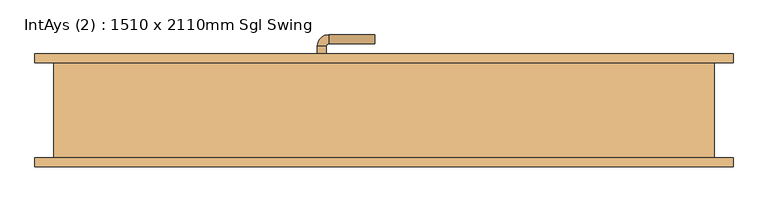
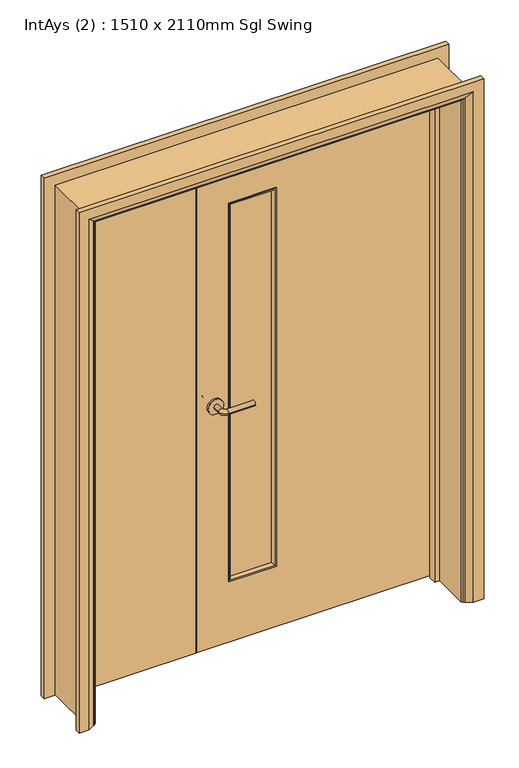
"""IFC4 building model written with IfcOpenShell, lengths in millimetres: door geometry, IntAys (2) : 1510 x 2110mm Sgl Swing."""

import ifcopenshell
import ifcopenshell.guid

model = None  # the IFC model being written
_history = None  # IfcOwnerHistory: only IFC2X3 demands one
_inside = {}  # id of a spatial element -> (the spatial element, [elements in it])
_under = {}  # id of a project, library or spatial element -> (it, [spatial elements below it])
_declared = {}  # id of a project -> (the project, [libraries it declares])
_typed = {}  # id of a type object -> (the type object, [elements of that type])
_made_of = {}  # id of a material, layer set ... -> (it, [elements and type objects made of it])


def new_model(schema):
    """Start an empty IFC model of exactly this schema.

    Asked for "IFC4X3", IfcOpenShell would pick the latest addendum, in which some entities
    have other attributes; the version numbers below select the first issue.
    IFC2X3 requires an IfcOwnerHistory on every rooted entity: one is made here for all.
    """
    global model, _history
    if schema == "IFC4X3":
        model = ifcopenshell.file(schema_version=(4, 3, 0, 0))
    else:
        model = ifcopenshell.file(schema=schema)
    _inside.clear()
    _under.clear()
    _declared.clear()
    _typed.clear()
    _made_of.clear()
    _history = None
    if model.schema == "IFC2X3":
        org = make("IfcOrganization", Name="unknown")
        user = make(
            "IfcPersonAndOrganization",
            ThePerson=make("IfcPerson", FamilyName="unknown"),
            TheOrganization=org,
        )
        app = make(
            "IfcApplication",
            ApplicationDeveloper=org,
            Version="unknown",
            ApplicationFullName="unknown",
            ApplicationIdentifier="unknown",
        )
        _history = make(
            "IfcOwnerHistory",
            OwningUser=user,
            OwningApplication=app,
            ChangeAction="ADDED",
            CreationDate=0,
        )
    return model


def make(cls, **values):
    """One entity of the class cls with the attributes given. An attribute that is None is left unset."""
    return model.create_entity(
        cls, **{name: value for name, value in values.items() if value is not None}
    )


def rooted(cls, **values):
    """An entity with a GlobalId (a new one), such as an element, a storey or a relation."""
    return make(cls, GlobalId=ifcopenshell.guid.new(), OwnerHistory=_history, **values)


def si_unit(unit_type, name, prefix=None):
    """IfcSIUnit, for example si_unit("LENGTHUNIT", "METRE", prefix="MILLI")."""
    return make("IfcSIUnit", UnitType=unit_type, Prefix=prefix, Name=name)


def assignment(units):
    """IfcUnitAssignment: the units of a project."""
    return None if units is None else make("IfcUnitAssignment", Units=units)


def point(xyz):
    """IfcCartesianPoint."""
    return None if xyz is None else make("IfcCartesianPoint", Coordinates=xyz)


def direction(xyz):
    """IfcDirection."""
    return None if xyz is None else make("IfcDirection", DirectionRatios=xyz)


def frame(location, z_axis=None, x_axis=None):
    """IfcAxis2Placement3D, a coordinate frame: its origin and axes. An axis left out is left unset."""
    return make(
        "IfcAxis2Placement3D",
        Location=point(location),
        Axis=direction(z_axis),
        RefDirection=direction(x_axis),
    )


def frame_2d(location, x_axis=None):
    """IfcAxis2Placement2D, a coordinate frame in the plane: its origin and x axis."""
    return make(
        "IfcAxis2Placement2D", Location=point(location), RefDirection=direction(x_axis)
    )


def origin():
    """The frame at (0, 0, 0) with its axes left unset."""
    return frame((0.0, 0.0, 0.0))


def place(relative_to, where):
    """IfcLocalPlacement: puts the frame where relative to a parent placement (None: the world)."""
    return make(
        "IfcLocalPlacement", PlacementRelTo=relative_to, RelativePlacement=where
    )


def context(
    kind, dimensions, precision=None, world=None, true_north=None, identifier=None
):
    """IfcGeometricRepresentationContext, for example the 3D "Model" context."""
    return make(
        "IfcGeometricRepresentationContext",
        ContextIdentifier=identifier,
        ContextType=kind,
        CoordinateSpaceDimension=dimensions,
        Precision=precision,
        WorldCoordinateSystem=world,
        TrueNorth=true_north,
    )


def project(units=None, contexts=None):
    """IfcProject with its units and contexts."""
    return rooted(
        "IfcProject",
        Name="project",
        RepresentationContexts=contexts,
        UnitsInContext=assignment(units),
    )


def spatial(cls, under=None, at=None, **own):
    """A site, building, storey or space (cls), placed at a placement, below another one or the project."""
    s = rooted(cls, ObjectPlacement=at, **own)
    if under is not None:
        _under.setdefault(under.id(), (under, []))[1].append(s)
    return s


def polyline(points):
    """IfcPolyline through the points."""
    return make("IfcPolyline", Points=[point(p) for p in points])


def circle_curve(where, radius):
    """IfcCircle in the frame where."""
    return make("IfcCircle", Position=where, Radius=radius)


def ellipse_curve(where, semi_axis1, semi_axis2):
    """IfcEllipse in the frame where."""
    return make(
        "IfcEllipse", Position=where, SemiAxis1=semi_axis1, SemiAxis2=semi_axis2
    )


def trimmed(basis, trim1, trim2, sense, master):
    """IfcTrimmedCurve: the piece of a basis curve between two trims."""
    return make(
        "IfcTrimmedCurve",
        BasisCurve=basis,
        Trim1=trim1,
        Trim2=trim2,
        SenseAgreement=sense,
        MasterRepresentation=master,
    )


def segment(curve, same_sense, transition):
    """IfcCompositeCurveSegment."""
    return make(
        "IfcCompositeCurveSegment",
        Transition=transition,
        SameSense=same_sense,
        ParentCurve=curve,
    )


def composite_curve(segments, self_intersect=None):
    """IfcCompositeCurve: segments joined end to end."""
    return make("IfcCompositeCurve", Segments=segments, SelfIntersect=self_intersect)


def outline(outer, holes=None, kind="AREA"):
    """IfcArbitraryClosedProfileDef: a profile drawn as a closed curve; with holes, ...WithVoids."""
    if holes is None:
        return make("IfcArbitraryClosedProfileDef", ProfileType=kind, OuterCurve=outer)
    return make(
        "IfcArbitraryProfileDefWithVoids",
        ProfileType=kind,
        OuterCurve=outer,
        InnerCurves=holes,
    )


def extrude(swept, where, along, depth):
    """IfcExtrudedAreaSolid: the profile swept, set in the frame where, extruded along a direction by depth."""
    return make(
        "IfcExtrudedAreaSolid",
        SweptArea=swept,
        Position=where,
        ExtrudedDirection=direction(along),
        Depth=depth,
    )


def faces_of(points, faces, orient=None, outer=None):
    """IfcFace entities. A face is a list of loops; a loop is a list of indices into points, from 0.

    orient and outer hold one flag for each loop. By default every Orientation is true, the
    first loop of a face is its IfcFaceOuterBound and the others are IfcFaceBound.
    """
    made = []
    for i, loops in enumerate(faces):
        bounds = []
        for j, loop in enumerate(loops):
            is_outer = j == 0 if outer is None else outer[i][j]
            bounds.append(
                make(
                    "IfcFaceOuterBound" if is_outer else "IfcFaceBound",
                    Bound=make("IfcPolyLoop", Polygon=[points[k] for k in loop]),
                    Orientation=True if orient is None else orient[i][j],
                )
            )
        made.append(make("IfcFace", Bounds=bounds))
    return made


def faceted_brep(points, faces, orient=None, outer=None, voids=None):
    """IfcFacetedBrep: a solid bounded by flat faces; with voids (closed shells), ...WithVoids."""
    shared = [point(p) for p in points]
    hull = make("IfcClosedShell", CfsFaces=faces_of(shared, faces, orient, outer))
    if voids is None:
        return make("IfcFacetedBrep", Outer=hull)
    return make(
        "IfcFacetedBrepWithVoids",
        Outer=hull,
        Voids=[
            make(cls, CfsFaces=faces_of(shared, fs, o, b)) for cls, fs, o, b in voids
        ],
    )


def shape(context_of_items, identifier, shape_type, items):
    """IfcShapeRepresentation: the items that make up one representation, for example the "Body"."""
    return make(
        "IfcShapeRepresentation",
        ContextOfItems=context_of_items,
        RepresentationIdentifier=identifier,
        RepresentationType=shape_type,
        Items=items,
    )


def source(mapping_origin, context_of_items, identifier, shape_type, items):
    """IfcRepresentationMap: a shape defined once, which mapped items show again and again."""
    return make(
        "IfcRepresentationMap",
        MappingOrigin=mapping_origin,
        MappedRepresentation=shape(context_of_items, identifier, shape_type, items),
    )


def transform(
    local_origin,
    x_axis=None,
    y_axis=None,
    z_axis=None,
    scale=None,
    scale2=None,
    scale3=None,
    uniform=True,
):
    """IfcCartesianTransformationOperator3D, or its non-uniform kind. x_axis, y_axis, z_axis: its Axis1, 2, 3."""
    if uniform:
        return make(
            "IfcCartesianTransformationOperator3D",
            Axis1=direction(x_axis),
            Axis2=direction(y_axis),
            LocalOrigin=point(local_origin),
            Scale=scale,
            Axis3=direction(z_axis),
        )
    return make(
        "IfcCartesianTransformationOperator3DnonUniform",
        Axis1=direction(x_axis),
        Axis2=direction(y_axis),
        LocalOrigin=point(local_origin),
        Scale=scale,
        Axis3=direction(z_axis),
        Scale2=scale2,
        Scale3=scale3,
    )


def mapped(mapping_source, mapping_target):
    """IfcMappedItem: shows the shape of a source again, moved by a transform."""
    return make(
        "IfcMappedItem", MappingSource=mapping_source, MappingTarget=mapping_target
    )


def made_of(thing, what):
    """Note that an element or type object is made of a material, layer set ...; save() writes the relation."""
    if what is not None:
        _made_of.setdefault(what.id(), (what, []))[1].append(thing)
    return thing


def element(
    cls,
    number,
    at=None,
    inside=None,
    cuts=None,
    type_object=None,
    material=None,
    context=None,
    identifier="Body",
    shape_type=None,
    held_by="IfcProductDefinitionShape",
    body=None,
    shapes=None,
    **own,
):
    """One element of the class cls, such as IfcWall. Its Tag is "e" and its number.

    at: its placement. inside: the storey or other place that contains it. cuts: it is an
    opening in that element (IfcRelVoidsElement). A single representation is given by context,
    identifier, shape_type and body (its items); several are given by shapes. held_by: the class
    of the entity that holds the representations. save() writes the other relations.
    """
    e = rooted(cls, Tag="e%d" % number, ObjectPlacement=at, **own)
    if body is not None:
        shapes = [shape(context, identifier, shape_type, body)]
    if shapes is not None:
        e.Representation = make(held_by, Representations=shapes)
    if inside is not None:
        _inside.setdefault(inside.id(), (inside, []))[1].append(e)
    if cuts is not None:
        rooted(
            "IfcRelVoidsElement", RelatingBuildingElement=cuts, RelatedOpeningElement=e
        )
    if type_object is not None:
        _typed.setdefault(type_object.id(), (type_object, []))[1].append(e)
    return made_of(e, material)


def aggregate(whole, parts):
    """IfcRelAggregates: a whole, such as a stair, and the parts it consists of."""
    return rooted("IfcRelAggregates", RelatingObject=whole, RelatedObjects=parts)


def save(model, path):
    """Write the relations noted so far, then the file.

    IfcRelAggregates (storeys below a building ...), IfcRelContainedInSpatialStructure (elements
    in a storey), IfcRelDefinesByType, IfcRelAssociatesMaterial and IfcRelDeclares: one each for
    every whole, place, type object, material and project.
    """
    for whole, parts in _under.values():
        aggregate(whole, parts)
    for where, things in _inside.values():
        rooted(
            "IfcRelContainedInSpatialStructure",
            RelatedElements=things,
            RelatingStructure=where,
        )
    for kind, things in _typed.values():
        rooted("IfcRelDefinesByType", RelatedObjects=things, RelatingType=kind)
    for what, things in _made_of.values():
        rooted("IfcRelAssociatesMaterial", RelatedObjects=things, RelatingMaterial=what)
    for by, libraries in _declared.values():
        rooted("IfcRelDeclares", RelatingContext=by, RelatedDefinitions=libraries)
    model.write(path)


def plane_surface(at):
    """IfcPlane: the flat surface through the origin of the frame at, square to its z axis."""
    return make("IfcPlane", Position=at)


def cylinder_surface(at, radius):
    """IfcCylindricalSurface: all points at the distance radius from the z axis of the frame at."""
    return make("IfcCylindricalSurface", Position=at, Radius=radius)


def revolved_surface(curve, axis_point, axis_direction):
    """IfcSurfaceOfRevolution: the curve turned about the line through axis_point along axis_direction."""
    return make(
        "IfcSurfaceOfRevolution",
        SweptCurve=make("IfcArbitraryOpenProfileDef", ProfileType="CURVE", Curve=curve),
        AxisPosition=make("IfcAxis1Placement", Location=point(axis_point), Axis=direction(axis_direction)),
    )


def advanced_brep(points, edges, surfaces, faces):
    """IfcAdvancedBrep: a solid bounded by faces that lie on surfaces and meet in shared edges.

    An edge is (start, end): straight between two places in points (the first is 0);
    or (start, end, curve); or (start, end, curve, False) where it runs against its curve.
    A face is (place in surfaces, loops), or (place, loops, False) where it looks against
    its surface's normal. A loop lists edges by number (the first is 1), with a minus sign
    where the edge is run from its end to its start. The first loop is the outer one.
    """
    corners = [point(p) for p in points]
    vertices = [make("IfcVertexPoint", VertexGeometry=c) for c in corners]
    made = []
    for start, end, *more in edges:
        made.append(
            make(
                "IfcEdgeCurve",
                EdgeStart=vertices[start],
                EdgeEnd=vertices[end],
                EdgeGeometry=more[0] if more else make("IfcPolyline", Points=[corners[start], corners[end]]),
                SameSense=more[1] if len(more) > 1 else True,
            )
        )
    hull = []
    for where, loops, *sense in faces:
        bounds = []
        for j, loop in enumerate(loops):
            ring = [make("IfcOrientedEdge", EdgeElement=made[abs(k) - 1], Orientation=k > 0) for k in loop]
            bounds.append(
                make(
                    "IfcFaceOuterBound" if j == 0 else "IfcFaceBound",
                    Bound=make("IfcEdgeLoop", EdgeList=ring),
                    Orientation=True,
                )
            )
        hull.append(make("IfcAdvancedFace", Bounds=bounds, FaceSurface=surfaces[where], SameSense=sense[0] if sense else True))
    return make("IfcAdvancedBrep", Outer=make("IfcClosedShell", CfsFaces=hull))


def intays_2_1510_x_2110mm_sgl_swing_d010f506(model_context):
    return source(origin(), model_context, "Body", "SolidModel", [
        advanced_brep(
        [(88.5, 67.5, 1000.0), (108.5, 67.5, 1000.0), (108.5, 37.5, 1000.0), (88.5, 37.5, 1000.0), (113.5, 32.5, 1000.0), (113.5, 12.5, 1000.0), (218.5, 12.5, 1000.0), (218.5, 32.5, 1000.0)],
        [
            (0, 1, circle_curve(frame((98.5, 67.5, 1000.0), z_axis=(0.0, 1.0, 0.0), x_axis=(1.0, 0.0, 0.0)), 10.0)),
            (1, 0, circle_curve(frame((98.5, 67.5, 1000.0), z_axis=(0.0, 1.0, 0.0), x_axis=(1.0, 0.0, 0.0)), 10.0)),
            (1, 2),
            (2, 3, circle_curve(frame((98.5, 37.5, 1000.0), z_axis=(0.0, 1.0, 0.0), x_axis=(1.0, 0.0, 0.0)), 10.0)),
            (3, 0),
            (3, 2, circle_curve(frame((98.5, 37.5, 1000.0), z_axis=(0.0, 1.0, 0.0), x_axis=(1.0, 0.0, 0.0)), 10.0)),
            (4, 5, circle_curve(frame((113.5, 22.5, 1000.0), z_axis=(-1.0, 0.0, 0.0), x_axis=(0.0, 1.0, 0.0)), 10.0)),
            (5, 3, circle_curve(frame((113.5, 37.5, 1000.0), z_axis=(0.0, 0.0, -1.0), x_axis=(-1.0, 0.0, 0.0)), 25.0)),
            (2, 4, circle_curve(frame((113.5, 37.5, 1000.0), z_axis=(0.0, 0.0, 1.0), x_axis=(-1.0, 0.0, 0.0)), 5.0)),
            (5, 4, circle_curve(frame((113.5, 22.5, 1000.0), z_axis=(-1.0, 0.0, 0.0), x_axis=(0.0, 1.0, 0.0)), 10.0)),
            (6, 7, circle_curve(frame((218.5, 22.5, 1000.0), z_axis=(1.0, 0.0, 0.0), x_axis=(0.0, 1.0, 0.0)), 10.0)),
            (7, 6, circle_curve(frame((218.5, 22.5, 1000.0), z_axis=(1.0, 0.0, 0.0), x_axis=(0.0, 1.0, 0.0)), 10.0)),
            (4, 7),
            (6, 5),
        ],
        [
            plane_surface(frame((98.5, 67.5, 1000.0), z_axis=(0.0, 1.0, 0.0), x_axis=(0.0, 0.0, 1.0))),
            cylinder_surface(frame((98.5, 67.5, 1000.0), z_axis=(0.0, 1.0, 0.0), x_axis=(1.0, 0.0, 0.0)), 10.0),
            revolved_surface(trimmed(ellipse_curve(frame((98.5, 37.5, 1000.0), z_axis=(0.0, -1.0, 0.0), x_axis=(1.0, 0.0, 0.0)), 10.0, 10.0), [point((88.5, 37.5, 1000.0))], [point((108.5, 37.5, 1000.0))], True, "CARTESIAN"), (113.5, 37.5, 1000.0), (0.0, 0.0, -1.0)),
            revolved_surface(trimmed(ellipse_curve(frame((98.5, 37.5, 1000.0), z_axis=(0.0, -1.0, 0.0), x_axis=(1.0, 0.0, 0.0)), 10.0, 10.0), [point((108.5, 37.5, 1000.0))], [point((88.5, 37.5, 1000.0))], True, "CARTESIAN"), (113.5, 37.5, 1000.0), (0.0, 0.0, -1.0)),
            plane_surface(frame((218.5, 22.5, 1000.0), z_axis=(1.0, 0.0, 0.0), x_axis=(0.0, 0.0, 1.0))),
            cylinder_surface(frame((113.5, 22.5, 1000.0), z_axis=(-1.0, 0.0, 0.0), x_axis=(0.0, 1.0, 0.0)), 10.0),
        ],
        [
            (0, [[1, 2]]),
            (1, [[3, 4, 5, -2]]),
            (1, [[-5, 6, -3, -1]]),
            (2, [[7, 8, -4, 9]]),
            (3, [[10, -9, -6, -8]]),
            (4, [[11, 12]]),
            (5, [[13, -11, 14, -7]]),
            (5, [[-14, -12, -13, -10]]),
        ],
    ),
        extrude(outline(composite_curve([segment(trimmed(circle_curve(frame_2d((1000.0, 96.0)), 30.0), [point((1000.0, 66.0))], [point((1000.0, 126.0))], False, "CARTESIAN"), True, "CONTINUOUS"), segment(trimmed(circle_curve(frame_2d((1000.0, 96.0)), 30.0), [point((1000.0, 126.0))], [point((1000.0, 66.0))], False, "CARTESIAN"), True, "CONTINUOUS")], self_intersect=False)), frame((0.0, 67.5, 0.0), z_axis=(0.0, 1.0, 0.0), x_axis=(0.0, 0.0, 1.0)), (0.0, 0.0, 1.0), 8.0),
        advanced_brep(
        [(88.5, 115.5, 1000.0), (108.5, 115.5, 1000.0), (88.5, 145.5, 1000.0), (108.5, 145.5, 1000.0), (113.5, 150.5, 1000.0), (113.5, 170.5, 1000.0), (218.5, 170.5, 1000.0), (218.5, 150.5, 1000.0)],
        [
            (0, 1, circle_curve(frame((98.5, 115.5, 1000.0), z_axis=(0.0, -1.0, 0.0), x_axis=(1.0, 0.0, 0.0)), 10.0)),
            (1, 0, circle_curve(frame((98.5, 115.5, 1000.0), z_axis=(0.0, -1.0, 0.0), x_axis=(1.0, 0.0, 0.0)), 10.0)),
            (0, 2),
            (2, 3, circle_curve(frame((98.5, 145.5, 1000.0), z_axis=(0.0, -1.0, 0.0), x_axis=(1.0, 0.0, 0.0)), 10.0)),
            (3, 1),
            (3, 2, circle_curve(frame((98.5, 145.5, 1000.0), z_axis=(0.0, -1.0, 0.0), x_axis=(1.0, 0.0, 0.0)), 10.0)),
            (4, 3, circle_curve(frame((113.5, 145.5, 1000.0), z_axis=(0.0, 0.0, 1.0), x_axis=(-1.0, 0.0, 0.0)), 5.0)),
            (2, 5, circle_curve(frame((113.5, 145.5, 1000.0), z_axis=(0.0, 0.0, -1.0), x_axis=(-1.0, 0.0, 0.0)), 25.0)),
            (5, 4, circle_curve(frame((113.5, 160.5, 1000.0), z_axis=(-1.0, 0.0, 0.0), x_axis=(0.0, -1.0, 0.0)), 10.0)),
            (4, 5, circle_curve(frame((113.5, 160.5, 1000.0), z_axis=(-1.0, 0.0, 0.0), x_axis=(0.0, -1.0, 0.0)), 10.0)),
            (6, 7, circle_curve(frame((218.5, 160.5, 1000.0), z_axis=(1.0, 0.0, 0.0), x_axis=(0.0, -1.0, 0.0)), 10.0)),
            (7, 6, circle_curve(frame((218.5, 160.5, 1000.0), z_axis=(1.0, 0.0, 0.0), x_axis=(0.0, -1.0, 0.0)), 10.0)),
            (5, 6),
            (7, 4),
        ],
        [
            plane_surface(frame((98.5, 115.5, 1000.0), z_axis=(0.0, -1.0, 0.0), x_axis=(0.0, 0.0, 1.0))),
            cylinder_surface(frame((98.5, 115.5, 1000.0), z_axis=(0.0, -1.0, 0.0), x_axis=(1.0, 0.0, 0.0)), 10.0),
            revolved_surface(trimmed(ellipse_curve(frame((98.5, 145.5, 1000.0), z_axis=(0.0, -1.0, 0.0), x_axis=(1.0, 0.0, 0.0)), 10.0, 10.0), [point((88.5, 145.5, 1000.0))], [point((108.5, 145.5, 1000.0))], True, "CARTESIAN"), (113.5, 145.5, 1000.0), (0.0, 0.0, -1.0)),
            revolved_surface(trimmed(ellipse_curve(frame((98.5, 145.5, 1000.0), z_axis=(0.0, -1.0, 0.0), x_axis=(1.0, 0.0, 0.0)), 10.0, 10.0), [point((108.5, 145.5, 1000.0))], [point((88.5, 145.5, 1000.0))], True, "CARTESIAN"), (113.5, 145.5, 1000.0), (0.0, 0.0, -1.0)),
            plane_surface(frame((218.5, 160.5, 1000.0), z_axis=(1.0, 0.0, 0.0), x_axis=(0.0, 0.0, 1.0))),
            cylinder_surface(frame((113.5, 160.5, 1000.0), z_axis=(-1.0, 0.0, 0.0), x_axis=(0.0, -1.0, 0.0)), 10.0),
        ],
        [
            (0, [[1, 2]]),
            (1, [[-1, 3, 4, 5]]),
            (1, [[-2, -5, 6, -3]]),
            (2, [[7, -4, 8, 9]]),
            (3, [[-8, -6, -7, 10]]),
            (4, [[11, 12]]),
            (5, [[-9, 13, -12, 14]]),
            (5, [[-10, -14, -11, -13]]),
        ],
    ),
        extrude(outline(composite_curve([segment(trimmed(circle_curve(frame_2d((1000.0, 96.0)), 30.0), [point((1000.0, 66.0))], [point((1000.0, 126.0))], False, "CARTESIAN"), True, "CONTINUOUS"), segment(trimmed(circle_curve(frame_2d((1000.0, 96.0)), 30.0), [point((1000.0, 126.0))], [point((1000.0, 66.0))], False, "CARTESIAN"), True, "CONTINUOUS")], self_intersect=False)), frame((0.0, 107.5, 0.0), z_axis=(0.0, 1.0, 0.0), x_axis=(0.0, 0.0, 1.0)), (0.0, 0.0, 1.0), 8.0),
        extrude(outline(polyline([(2102.0, -508.0), (0.0, -508.0), (0.0, -476.0), (2070.0, -476.0), (2070.0, 954.0), (0.0, 954.0), (0.0, 986.0), (2102.0, 986.0), (2102.0, -508.0)])), frame((0.0, -107.5, 0.0), z_axis=(0.0, 1.0, 0.0), x_axis=(0.0, 0.0, 1.0)), (0.0, 0.0, 1.0), 215.0),
        advanced_brep(
        [(-551.0, -127.5, 0.0), (-551.0, -107.5, 0.0), (-481.0, -107.5, 0.0), (-485.0, -113.5, 0.0), (-511.0, -127.5, 0.0), (-551.0, -127.5, 2145.0), (-551.0, -107.5, 2145.0), (1029.0, -107.5, 2145.0), (1029.0, -107.5, 0.0), (959.0, -107.5, 0.0), (959.0, -107.5, 2075.0), (-481.0, -107.5, 2075.0), (-485.0, -113.5, 2079.0), (-511.0, -127.5, 2105.0), (989.0, -127.5, 2105.0), (989.0, -127.5, 0.0), (1029.0, -127.5, 0.0), (1029.0, -127.5, 2145.0), (963.0, -113.5, 0.0), (963.0, -113.5, 2079.0)],
        [
            (0, 1),
            (1, 2),
            (2, 3, circle_curve(frame((-489.0, -106.5, 0.0), z_axis=(0.0, 0.0, -1.0), x_axis=(-1.0, 0.0, 0.0)), 8.0622577)),
            (3, 4),
            (4, 0),
            (0, 5),
            (5, 6),
            (6, 1),
            (6, 7),
            (7, 8),
            (8, 9),
            (9, 10),
            (10, 11),
            (11, 2),
            (11, 12, ellipse_curve(frame((-489.0, -106.5, 2083.0), z_axis=(-0.7071067811865475, 0.0, -0.7071067811865475), x_axis=(0.7071067811865474, 0.0, -0.7071067811865476)), 11.4017543, 8.0622577)),
            (12, 3),
            (12, 13),
            (13, 4),
            (13, 14),
            (14, 15),
            (15, 16),
            (16, 17),
            (17, 5),
            (7, 17),
            (16, 8),
            (15, 18),
            (18, 9, circle_curve(frame((967.0, -106.5, 0.0), z_axis=(0.0, 0.0, -1.0), x_axis=(1.0, 0.0, 0.0)), 8.0622577)),
            (19, 10, ellipse_curve(frame((967.0, -106.5, 2083.0), z_axis=(0.7071067811865475, 0.0, -0.7071067811865475), x_axis=(0.7071067811865474, 0.0, 0.7071067811865476)), 11.4017543, 8.0622577)),
            (18, 19),
            (14, 19),
            (19, 12),
        ],
        [
            plane_surface(frame((-481.0, -107.5, 0.0), z_axis=(0.0, 0.0, -1.0), x_axis=(0.0, -1.0, 0.0))),
            plane_surface(frame((-551.0, -127.5, 0.0), z_axis=(-1.0, 0.0, 0.0), x_axis=(0.0, 0.0, 1.0))),
            plane_surface(frame((-551.0, -107.5, 0.0), z_axis=(0.0, 1.0, 0.0), x_axis=(0.0, 0.0, 1.0))),
            cylinder_surface(frame((-489.0, -106.5, 0.0), z_axis=(0.0, 0.0, -1.0), x_axis=(-1.0, 0.0, 0.0)), 8.0622577),
            plane_surface(frame((-485.0, -113.5, 0.0), z_axis=(0.4740998230350183, -0.8804710999221749, 0.0), x_axis=(0.0, 0.0, 1.0))),
            plane_surface(frame((-511.0, -127.5, 0.0), z_axis=(0.0, -1.0, 0.0), x_axis=(0.0, 0.0, 1.0))),
            plane_surface(frame((1029.0, -127.5, 2145.0), z_axis=(1.0, 0.0, 0.0), x_axis=(0.0, 0.0, -1.0))),
            plane_surface(frame((959.0, -107.5, 0.0), z_axis=(0.0, 0.0, -1.0), x_axis=(0.0, -1.0, 0.0))),
            cylinder_surface(frame((967.0, -106.5, 2075.0), z_axis=(0.0, 0.0, 1.0), x_axis=(1.0, 0.0, 0.0)), 8.0622577),
            plane_surface(frame((963.0, -113.5, 2079.0), z_axis=(-0.4740998230350183, -0.8804710999221749, 0.0), x_axis=(0.0, 0.0, -1.0))),
            plane_surface(frame((-551.0, -127.5, 2145.0), z_axis=(0.0, 0.0, 1.0), x_axis=(1.0, 0.0, 0.0))),
            cylinder_surface(frame((-481.0, -106.5, 2083.0), z_axis=(-1.0, 0.0, 0.0), x_axis=(0.0, 0.0, 1.0)), 8.0622577),
            plane_surface(frame((-485.0, -113.5, 2079.0), z_axis=(0.0, -0.8804710999221749, -0.4740998230350183), x_axis=(1.0, 0.0, 0.0))),
        ],
        [
            (0, [[1, 2, 3, 4, 5]]),
            (1, [[-1, 6, 7, 8]]),
            (2, [[-2, -8, 9, 10, 11, 12, 13, 14]]),
            (3, [[-3, -14, 15, 16]]),
            (4, [[-4, -16, 17, 18]]),
            (5, [[-5, -18, 19, 20, 21, 22, 23, -6]]),
            (6, [[24, -22, 25, -10]]),
            (7, [[-21, 26, 27, -11, -25]]),
            (8, [[28, -12, -27, 29]]),
            (9, [[30, -29, -26, -20]]),
            (10, [[-7, -23, -24, -9]]),
            (11, [[-15, -13, -28, 31]]),
            (12, [[-17, -31, -30, -19]]),
        ],
    ),
        advanced_brep(
        [(1029.0, 127.5, 0.0), (1029.0, 107.5, 0.0), (959.0, 107.5, 0.0), (963.0, 113.5, 0.0), (989.0, 127.5, 0.0), (1029.0, 127.5, 2145.0), (1029.0, 107.5, 2145.0), (-551.0, 107.5, 2145.0), (-551.0, 107.5, 0.0), (-481.0, 107.5, 0.0), (-481.0, 107.5, 2075.0), (959.0, 107.5, 2075.0), (963.0, 113.5, 2079.0), (989.0, 127.5, 2105.0), (-511.0, 127.5, 2105.0), (-511.0, 127.5, 0.0), (-551.0, 127.5, 0.0), (-551.0, 127.5, 2145.0), (-485.0, 113.5, 0.0), (-485.0, 113.5, 2079.0)],
        [
            (0, 1),
            (1, 2),
            (2, 3, circle_curve(frame((967.0, 106.5, 0.0), z_axis=(0.0, 0.0, -1.0), x_axis=(1.0, 0.0, 0.0)), 8.0622577)),
            (3, 4),
            (4, 0),
            (0, 5),
            (5, 6),
            (6, 1),
            (6, 7),
            (7, 8),
            (8, 9),
            (9, 10),
            (10, 11),
            (11, 2),
            (11, 12, ellipse_curve(frame((967.0, 106.5, 2083.0), z_axis=(0.7071067811865475, 0.0, -0.7071067811865475), x_axis=(-0.7071067811865474, 0.0, -0.7071067811865476)), 11.4017543, 8.0622577)),
            (12, 3),
            (12, 13),
            (13, 4),
            (13, 14),
            (14, 15),
            (15, 16),
            (16, 17),
            (17, 5),
            (7, 17),
            (16, 8),
            (15, 18),
            (18, 9, circle_curve(frame((-489.0, 106.5, 0.0), z_axis=(0.0, 0.0, -1.0), x_axis=(-1.0, 0.0, 0.0)), 8.0622577)),
            (19, 10, ellipse_curve(frame((-489.0, 106.5, 2083.0), z_axis=(-0.7071067811865475, 0.0, -0.7071067811865475), x_axis=(-0.7071067811865474, 0.0, 0.7071067811865476)), 11.4017543, 8.0622577)),
            (18, 19),
            (14, 19),
            (19, 12),
        ],
        [
            plane_surface(frame((959.0, 107.5, 0.0), z_axis=(0.0, 0.0, -1.0), x_axis=(0.0, -1.0, 0.0))),
            plane_surface(frame((1029.0, 127.5, 0.0), z_axis=(1.0, 0.0, 0.0), x_axis=(0.0, 0.0, 1.0))),
            plane_surface(frame((1029.0, 107.5, 0.0), z_axis=(0.0, -1.0, 0.0), x_axis=(0.0, 0.0, 1.0))),
            cylinder_surface(frame((967.0, 106.5, 0.0), z_axis=(0.0, 0.0, -1.0), x_axis=(1.0, 0.0, 0.0)), 8.0622577),
            plane_surface(frame((963.0, 113.5, 0.0), z_axis=(-0.4740998230350126, 0.8804710999221779, 0.0), x_axis=(0.0, 0.0, 1.0))),
            plane_surface(frame((989.0, 127.5, 0.0), z_axis=(0.0, 1.0, 0.0), x_axis=(0.0, 0.0, 1.0))),
            plane_surface(frame((-551.0, 127.5, 2145.0), z_axis=(-1.0, 0.0, 0.0), x_axis=(0.0, 0.0, -1.0))),
            plane_surface(frame((-481.0, 107.5, 0.0), z_axis=(0.0, 0.0, -1.0), x_axis=(0.0, -1.0, 0.0))),
            cylinder_surface(frame((-489.0, 106.5, 2075.0), z_axis=(0.0, 0.0, 1.0), x_axis=(-1.0, 0.0, 0.0)), 8.0622577),
            plane_surface(frame((-485.0, 113.5, 2079.0), z_axis=(0.4740998230350183, 0.8804710999221749, 0.0), x_axis=(0.0, 0.0, -1.0))),
            plane_surface(frame((1029.0, 127.5, 2145.0), z_axis=(0.0, 0.0, 1.0), x_axis=(-1.0, 0.0, 0.0))),
            cylinder_surface(frame((959.0, 106.5, 2083.0), z_axis=(1.0, 0.0, 0.0), x_axis=(0.0, 0.0, 1.0)), 8.0622577),
            plane_surface(frame((963.0, 113.5, 2079.0), z_axis=(0.0, 0.8804710999221763, -0.4740998230350154), x_axis=(-1.0, 0.0, 0.0))),
        ],
        [
            (0, [[1, 2, 3, 4, 5]]),
            (1, [[-1, 6, 7, 8]]),
            (2, [[-2, -8, 9, 10, 11, 12, 13, 14]]),
            (3, [[-3, -14, 15, 16]]),
            (4, [[-4, -16, 17, 18]]),
            (5, [[-5, -18, 19, 20, 21, 22, 23, -6]]),
            (6, [[24, -22, 25, -10]]),
            (7, [[-21, 26, 27, -11, -25]]),
            (8, [[28, -12, -27, 29]]),
            (9, [[30, -29, -26, -20]]),
            (10, [[-7, -23, -24, -9]]),
            (11, [[-15, -13, -28, 31]]),
            (12, [[-17, -31, -30, -19]]),
        ],
    ),
        faceted_brep([(-457.0, 72.5, 0.0), (-457.0, 40.5, 0.0), (-476.0, 40.5, 0.0), (-476.0, 72.5, 0.0), (-457.0, 72.5, 2051.0), (-457.0, 40.5, 2051.0), (-476.0, 40.5, 2070.0), (-476.0, 72.5, 2070.0), (935.0, 72.5, 0.0), (954.0, 72.5, 0.0), (954.0, 40.5, 0.0), (935.0, 40.5, 0.0), (935.0, 72.5, 2051.0), (954.0, 72.5, 2070.0), (954.0, 40.5, 2070.0), (935.0, 40.5, 2051.0)], [[[0, 1, 2, 3]], [[1, 0, 4, 5]], [[2, 1, 5, 6]], [[3, 2, 6, 7]], [[0, 3, 7, 4]], [[8, 9, 10, 11]], [[12, 13, 9, 8]], [[13, 14, 10, 9]], [[14, 15, 11, 10]], [[15, 12, 8, 11]], [[5, 4, 12, 15]], [[6, 5, 15, 14]], [[7, 6, 14, 13]], [[4, 7, 13, 12]]]),
        extrude(outline(polyline([(335.0, 85.5), (150.0, 85.5), (150.0, 97.5), (335.0, 97.5), (335.0, 85.5)])), frame((0.0, 0.0, 257.0), z_axis=(0.0, 0.0, 1.0), x_axis=(1.0, 0.0, 0.0)), (0.0, 0.0, 1.0), 1560.0),
        extrude(outline(polyline([(22.0, 75.5), (-473.0, 75.5), (-473.0, 107.5), (22.0, 107.5), (22.0, 75.5)])), frame((0.0, 0.0, 5.753223), z_axis=(0.0, 0.0, 1.0), x_axis=(1.0, 0.0, 0.0)), (0.0, 0.0, 1.0), 2061.246777),
        extrude(outline(polyline([(5.753223, 951.0), (2067.0, 951.0), (2067.0, 25.0), (5.753223, 25.0), (5.753223, 951.0)]), holes=[polyline([(1817.0, 150.0), (1817.0, 335.0), (257.0, 335.0), (257.0, 150.0), (1817.0, 150.0)])]), frame((0.0, 75.5, 0.0), z_axis=(0.0, 1.0, 0.0), x_axis=(0.0, 0.0, 1.0)), (0.0, 0.0, 1.0), 32.0),
        faceted_brep([(335.0, 72.5, 257.0), (335.0, 85.5, 257.0), (335.0, 85.5, 1817.0), (335.0, 72.5, 1817.0), (323.0, 85.5, 269.0), (329.0, 72.5, 263.0), (329.0, 72.5, 1811.0), (323.0, 85.5, 1805.0), (150.0, 85.5, 1817.0), (150.0, 72.5, 1817.0), (156.0, 72.5, 1811.0), (162.0, 85.5, 1805.0), (150.0, 85.5, 257.0), (150.0, 72.5, 257.0), (156.0, 72.5, 263.0), (162.0, 85.5, 269.0)], [[[0, 1, 2, 3]], [[4, 5, 6, 7]], [[3, 2, 8, 9]], [[7, 6, 10, 11]], [[9, 8, 12, 13]], [[11, 10, 14, 15]], [[1, 12, 8, 2], [7, 11, 15, 4]], [[13, 12, 1, 0]], [[3, 9, 13, 0], [5, 14, 10, 6]], [[15, 14, 5, 4]]]),
        faceted_brep([(150.0, 110.5, 257.0), (150.0, 97.5, 257.0), (150.0, 97.5, 1817.0), (150.0, 110.5, 1817.0), (162.0, 97.5, 269.0), (156.0, 110.5, 263.0), (156.0, 110.5, 1811.0), (162.0, 97.5, 1805.0), (335.0, 97.5, 1817.0), (335.0, 110.5, 1817.0), (329.0, 110.5, 1811.0), (323.0, 97.5, 1805.0), (335.0, 97.5, 257.0), (335.0, 110.5, 257.0), (329.0, 110.5, 263.0), (323.0, 97.5, 269.0)], [[[0, 1, 2, 3]], [[4, 5, 6, 7]], [[3, 2, 8, 9]], [[7, 6, 10, 11]], [[9, 8, 12, 13]], [[11, 10, 14, 15]], [[1, 12, 8, 2], [7, 11, 15, 4]], [[13, 12, 1, 0]], [[3, 9, 13, 0], [5, 14, 10, 6]], [[15, 14, 5, 4]]]),
    ])


if __name__ == "__main__":
    model = new_model("IFC4")
    model_context = context("Model", 3, world=origin())
    ifc_project = project(units=[si_unit("LENGTHUNIT", "METRE", prefix="MILLI")], contexts=[model_context])
    site = spatial("IfcSite", under=ifc_project)
    building = spatial("IfcBuilding", under=site)
    placement = place(None, origin())
    intays_2_1510_x_2110mm_sgl_swing_shape = intays_2_1510_x_2110mm_sgl_swing_d010f506(model_context)
    element("IfcDoor", 1, ObjectType="IntAys (2) : 1510 x 2110mm Sgl Swing", at=placement, inside=building, context=model_context, shape_type="MappedRepresentation", body=[
        mapped(intays_2_1510_x_2110mm_sgl_swing_shape, transform((0.0, 0.0, 0.0), x_axis=(1.0, 0.0, 0.0), y_axis=(0.0, 1.0, 0.0), z_axis=(0.0, 0.0, 1.0))),
    ])
    save(model, "model.ifc")

# Revit data of these elements
# Type "IntAys (2) : 1510 x 2110mm Sgl Swing"
#   Type Mark = "46"
#   Type Comments = "Internal Asymmetric"
#   Operation = "DoubleDoorSingleSwing"
#   Construction Type Id = "SGL"
#   Keynote = "L20"
#   Description = "Internal Asymmetric Door"
#   Analytic Construction = "Large single-glazed windows"
#   Visual Light Transmittance = 0.9
#   VisionPanel Width = 185 mm
#   Thickness = 32 mm
#   Stop Thickness = 19 mm
#   Stop Depth = 32 mm
#   Stile Top Rail = 250 mm
#   Stile Shutting = 125 mm
#   Stile Bottom Rail = 250 mm
#   Solar Heat Gain Coefficient = 0.86
#   Secondary Panel Width = 495 mm
#   Rough Width = 1510 mm
#   Rough Height = 2110 mm
#   Main Panel Width = 926 mm
#   Heat Transfer Coefficient (U) = 5.5617 W/(m²·K)
#   Handle Z Distance = 1000 mm
#   Handle X Distance = 75 mm
#   Handle Length = 350 mm
#   Frame Thickness = 32 mm
#   Door Panel Width = 926 mm
#   Door Panel Thickness = 32 mm
#   Height = 2110 mm
#   Door Panel Offset = 0 mm
#   Structural Tolerance = 8 mm
#   Tolerance = 3 mm
#   UnderCut = 7 mm
#   Width = 1510 mm
#   Door Panel Height = 2060 mm
#   Architrave Setback = 5 mm
#   Vis - Swing Single = yes
#   Vis - Swing Opposing = no
#   Vis - Swing Double = no
#   Vis - Stops = yes
#   Vis - Ironmongery = yes
#   Define Thermal Properties by = 1
#   Material Ironmongery = Door - Handle
#   Material Glass = Door - Glazing
#   Material Frame = Door - Frame/Mullion
#   Material Door = Door - Panel
#   Material Beading = Door - Panel
#   Material Architrave = Door - Architrave
#   Handle Style = element 261135
#   Function = (empty or 0)
#   Wall Closure = (empty or 0)
# Element 1 (IfcDoor, "IntAys (2) : 1510 x 2110mm Sgl Swing")
#   Materials on its faces: "Door - Panel", "Door - Architrave", "Door - Handle", "Door - Frame/Mullion", "Door - Glazing"
# Materials
#   "Door - Handle": class "Miscellaneous", colour RGB 0 0 0, transparency 0, Keynote = "P21"
#   "Door - Glazing": class "Miscellaneous", colour RGB 0 0 255, transparency 0.75
#   "Door - Frame/Mullion": class "Wood", colour RGB 212 179 113, transparency 0, Keynote = "L20"
#   "Door - Panel": class "Wood", colour RGB 210 159 95, transparency 0, Keynote = "L20"
#   "Door - Architrave": class "Wood", colour RGB 154 90 5, transparency 0, Keynote = "P20"
